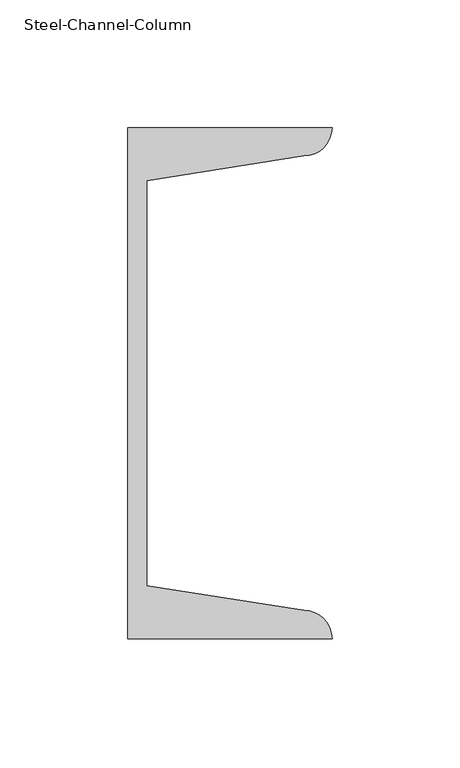
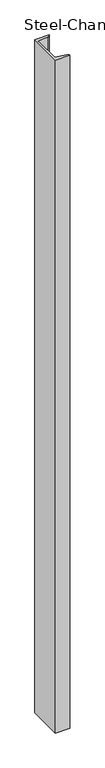
# IFC4 building model written with IfcOpenShell, lengths in millimetres: column geometry, Steel-Channel-Column : CL126_C-200×80x7.5x11.
# Revit data of these elements (continued)
# Project information (continued)
#     -cfd758078946\" /><element revit_id=\"af7cfdda-f71a-4a09-bb03-63e0c16d5d93-001530cf\" ism_id=\"46a5ded9-4fed-43a0-a06e-bb0fce603002\" /><element revit_id=\"af7cfdda-f71a-4a09-bb03-63e0c16d5d93-001530d1\" ism_id=\"62d05a0c-55f2-4c29-a355-b77f91c84c50\" /><element revit_id=\"af7cfdda-f71a-4a09-bb03-63e0c16d5d93-001530d3\" ism_id=\"eac0c420-7041-45a3-ad98-0cab4f5d8155\" /><element revit_id=\"af7cfdda-f71a-4a09-bb03-63e0c16d5d93-001530d5\" ism_id=\"9f5beb51-429a-4c7b-aa2e-ad2efe601ed6\" /><element revit_id=\"af7cfdda-f71a-4a09-bb03-63e0c16d5d93-001530d7\" ism_id=\"4613af3e-a189-4781-a937-106d789655c9\" /><element revit_id=\"af7cfdda-f71a-4a09-bb03-63e0c16d5d93-001530d9\" ism_id=\"71402e21-51c1-43b7-b8cc-75d2aba247eb\" /><element revit_id=\"af7cfdda-f71a-4a09-bb03-63e0c16d5d93-001530db\" ism_id=\"89101b83-9b84-4f11-b026-90cd564a3900\" /><element revit_id=\"af7cfdda-f71a-4a09-bb03-63e0c16d5d93-001530dd\" ism_id=\"37670781-ce23-4ce1-992b-7a400613c37b\" /><element revit_id=\"af7cfdda-f71a-4a09-bb03-63e0c16d5d93-001530df\" ism_id=\"2316856d-18eb-466b-8ab8-114816378db0\" /><element revit_id=\"af7cfdda-f71a-4a09-bb03-63e0c16d5d93-001530e2\" ism_id=\"da4f1597-5b5a-43a6-aa94-e478ffd6cfc7\" /><element revit_id=\"af7cfdda-f71a-4a09-bb03-63e0c16d5d93-001530e5\" ism_id=\"60805764-efb2-4434-8d81-aed3c3ed3c1b\" /><element revit_id=\"af7cfdda-f71a-4a09-bb03-63e0c16d5d93-001530e8\" ism_id=\"34e34ebb-6481-4bfb-b3d0-cb52295ff652\" /><element revit_id=\"af7cfdda-f71a-4a09-bb03-63e0c16d5d93-001530eb\" ism_id=\"dd5c4d73-1406-4c40-a955-5f9c52d01161\" /><element revit_id=\"af7cfdda-f71a-4a09-bb03-63e0c16d5d93-001530ed\" ism_id=\"cf8abc6b-638f-4bd5-8b66-615be032e220\" /><element revit_id=\"af7cfdda-f71a-4a09-bb03-63e0c16d5d93-001530f0\" ism_id=\"56ce8857-0c24-48d5-82f2-459e263998e2\" /><element revit_id=\"af7cfdda-f71a-4a09-bb03-63e0c16d5d93-001530f2\" ism_id=\"a1f000e8-ea08-442b-8a96-da7657653fd5\" /><element revit_id=\"af7cfdda-f71a-4a09-bb03-63e0c16d5d93-001530f4\" ism_id=\"2625e954-f7fb-41eb-b9bd-1b615ef945fc\" /><element revit_id=\"af7cfdda-f71a-4a09-bb03-63e0c16d5d93-001530f6\" ism_id=\"48469362-393c-4deb-bbb2-ad00180a23fb\" /><element revit_id=\"af7cfdda-f71a-4a09-bb03-63e0c16d5d93-001530f8\" ism_id=\"8e650f6f-0906-45a9-8fb8-35680155d6db\" /><element revit_id=\"af7cfdda-f71a-4a09-bb03-63e0c16d5d93-001530fb\" ism_id=\"f84acaf6-20a1-4df6-afed-1dc07fd0b2e9\" /><element revit_id=\"af7cfdda-f71a-4a09-bb03-63e0c16d5d93-001530fe\" ism_id=\"72816c7e-9128-47f4-b46a-ee567a2a03d6\" /><element revit_id=\"af7cfdda-f71a-4a09-bb03-63e0c16d5d93-00153100\" ism_id=\"c95ab0f8-b4bf-4b7c-bd1d-0423c8ac725a\" /><element revit_id=\"af7cfdda-f71a-4a09-bb03-63e0c16d5d93-00153102\" ism_id=\"32fd4119-6673-4973-aef2-b39ef90310e5\" /><element revit_id=\"af7cfdda-f71a-4a09-bb03-63e0c16d5d93-00153104\" ism_id=\"fd2aa4a6-d123-4100-85b9-db27c20cf6bc\" /><element revit_id=\"af7cfdda-f71a-4a09-bb03-63e0c16d5d93-00153106\" ism_id=\"e00fdefa-e77c-4406-9dbe-3c9122259821\" /><element revit_id=\"af7cfdda-f71a-4a09-bb03-63e0c16d5d93-00153108\" ism_id=\"25e5b79e-07c2-4ffa-a7a9-bf039dd2ad78\" /><element revit_id=\"af7cfdda-f71a-4a09-bb03-63e0c16d5d93-0015310b\" ism_id=\"720021d4-ca74-47c0-9c64-7d0854fa39f5\" /><element revit_id=\"af7cfdda-f71a-4a09-bb03-63e0c16d5d93-0015310d\" ism_id=\"ea922120-0cff-4f8d-a5c2-2841c031873e\" /><element revit_id=\"af7cfdda-f71a-4a09-bb03-63e0c16d5d93-0015310f\" ism_id=\"9d07ca73-3a65-44fe-ab61-476d8d1352d1\" /><element revit_id=\"af7cfdda-f71a-4a09-bb03-63e0c16d5d93-00153111\" ism_id=\"68a2fb30-d213-40c7-a166-dad5a20bd269\" /><element revit_id=\"af7cfdda-f71a-4a09-bb03-63e0c16d5d93-00153113\" ism_id=\"06119775-28f9-44f0-a265-5c57029016d1\" /><element revit_id=\"af7cfdda-f71a-4a09-bb03-63e0c16d5d93-00153115\" ism_id=\"ca133383-8253-4d07-aa92-f507fbb2ee47\" /><element revit_id=\"af7cfdda-f71a-4a09-bb03-63e0c16d5d93-00153117\" ism_id=\"6f4a7c07-4bd3-4c99-b1e4-110c964ccc07\" /><element revit_id=\"af7cfdda-f71a-4a09-bb03-63e0c16d5d93-00153119\" ism_id=\"ee1f865b-98a9-4ff1-a84c-52926e8f3566\" /><element revit_id=\"af7cfdda-f71a-4a09-bb03-63e0c16d5d93-0015311b\" ism_id=\"4fd7bd5c-7c46-4e79-a72b-dab4a1d98f33\" /><element revit_id=\"af7cfdda-f71a-4a09-bb03-63e0c16d5d93-0015311e\" ism_id=\"9ca0cac6-aaff-412a-b9c1-a8be985bc44a\" /><element revit_id=\"af7cfdda-f71a-4a09-bb03-63e0c16d5d93-00153121\" ism_id=\"73123639-76b5-46f0-a49e-b26af36d93b1\" /><element revit_id=\"af7cfdda-f71a-4a09-bb03-63e0c16d5d93-00153123\" ism_id=\"f74e8cb9-a93d-4aaa-985b-c0ed9befad19\" /><element revit_id=\"af7cfdda-f71a-4a09-bb03-63e0c16d5d93-00153126\" ism_id=\"5778daa1-b4cb-4cc3-9b7d-323562a47fba\" /><element revit_id=\"af7cfdda-f71a-4a09-bb03-63e0c16d5d93-00153129\" ism_id=\"2d7457d2-8978-4c95-9056-ebbaed3263eb\" /><element revit_id=\"af7cfdda-f71a-4a09-bb03-63e0c16d5d93-0015312c\" ism_id=\"48b420ce-6767-430a-aadc-695c25361a2d\" /><element revit_id=\"af7cfdda-f71a-4a09-bb03-63e0c16d5d93-0015312e\" ism_id=\"fc34038c-136d-4d55-b951-9cc35899fd33\" /><element revit_id=\"af7cfdda-f71a-4a09-bb03-63e0c16d5d93-00153130\" ism_id=\"e7a25938-3b91-4519-a48d-86fdd79489d5\" /><element revit_id=\"af7cfdda-f71a-4a09-bb03-63e0c16d5d93-00153133\" ism_id=\"c81dfd8c-579c-4d77-ab89-bf1f415d9cc6\" /><element revit_id=\"af7cfdda-f71a-4a09-bb03-63e0c16d5d93-00153136\" ism_id=\"5756a4b4-84ca-418c-b9f6-2d2370afca2f\" /><element revit_id=\"af7cfdda-f71a-4a09-bb03-63e0c16d5d93-0015313a\" ism_id=\"09a9cede-a757-4d8e-a722-6140af98bc61\" /><element revit_id=\"af7cfdda-f71a-4a09-bb03-63e0c16d5d93-0015313d\" ism_id=\"ac9b583c-7f63-4351-8b69-3967279b234c\" /><element revit_id=\"af7cfdda-f71a-4a09-bb03-63e0c16d5d93-00153140\" ism_id=\"1a52584d-6b21-4de6-bb42-5b9bdd6f24e9\" /><element revit_id=\"af7cfdda-f71a-4a09-bb03-63e0c16d5d93-00153143\" ism_id=\"6c2e2bc0-8432-4c98-9292-cbb2182bd4b0\" /><element revit_id=\"af7cfdda-f71a-4a09-bb03-63e0c16d5d93-00153145\" ism_id=\"644bb900-7654-42c5-a9b7-996a2197f6d0\" /><element revit_id=\"af7cfdda-f71a-4a09-bb03-63e0c16d5d93-00153148\" ism_id=\"a1bca0bd-75db-464c-b27a-2a69d9b4ad3d\" /><element revit_id=\"af7cfdda-f71a-4a09-bb03-63e0c16d5d93-0015314a\" ism_id=\"ea29955b-34f2-409a-aefa-e6adfe75349e\" /><element revit_id=\"af7cfdda-f71a-4a09-bb03-63e0c16d5d93-0015314d\" ism_id=\"800fef33-e5e1-422c-b708-e9394bbeefcc\" /><element revit_id=\"af7cfdda-f71a-4a09-bb03-63e0c16d5d93-0015314f\" ism_id=\"86259dca-8773-4253-ac56-e71252267c8a\" /><element revit_id=\"af7cfdda-f71a-4a09-bb03-63e0c16d5d93-00153152\" ism_id=\"d15a0ad2-db9f-420d-bea3-41a78a0eb330\" /><element revit_id=\"af7cfdda-f71a-4a09-bb03-63e0c16d5d93-00153155\" ism_id=\"bd27f420-df49-4abe-bd96-8e48e7f4efcb\" /><element revit_id=\"af7cfdda-f71a-4a09-bb03-63e0c16d5d93-00153157\" ism_id=\"5d451f94-860d-4cc3-a4fa-51a9f3126e33\" /><element revit_id=\"af7cfdda-f71a-4a09-bb03-63e0c16d5d93-0015315a\" ism_id=\"4234158a-994a-492b-85da-6108709b7232\" /><element revit_id=\"af7cfdda-f71a-4a09-bb03-63e0c16d5d93-0015315c\" ism_id=\"ca24c92d-986b-417f-812f-024ab15e24c8\" /><element revit_id=\"af7cfdda-f71a-4a09-bb03-63e0c16d5d93-0015315f\" ism_id=\"699ec3b0-0151-4110-b054-14418651f324\" /><element revit_id=\"af7cfdda-f71a-4a09-bb03-63e0c16d5d93-00153161\" ism_id=\"38ecdeac-3d85-48dd-82c1-53fe93f49beb\" /><element revit_id=\"af7cfdda-f71a-4a09-bb03-63e0c16d5d93-00153163\" ism_id=\"1340aefd-b79c-4264-8a49-d0a0504eff8c\" /><element revit_id=\"af7cfdda-f71a-4a09-bb03-63e0c16d5d93-00153165\" ism_id=\"1b6167c2-fb26-4b8d-916b-d835d89896e7\" /><element revit_id=\"af7cfdda-f71a-4a09-bb03-63e0c16d5d93-00153167\" ism_id=\"290d3d83-57eb-4125-aecb-a977a5fcf5ca\" /><element revit_id=\"af7cfdda-f71a-4a09-bb03-63e0c16d5d93-00153169\" ism_id=\"105c9b97-1c70-4237-82ac-8404a3e8e6a6\" /><element revit_id=\"af7cfdda-f71a-4a09-bb03-63e0c16d5d93-0015316c\" ism_id=\"1726c5bb-05e2-4959-9da2-4227f0219f00\" /><element revit_id=\"af7cfdda-f71a-4a09-bb03-63e0c16d5d93-0015316e\" ism_id=\"d919ee9c-caed-4119-b451-e3644db952c8\" /><element revit_id=\"af7cfdda-f71a-4a09-bb03-63e0c16d5d93-00153170\" ism_id=\"1b1fab26-60c4-40ed-b31b-b177eda246ce\" /><element revit_id=\"af7cfdda-f71a-4a09-bb03-63e0c16d5d93-00153172\" ism_id=\"ea9b5221-a1f2-4796-8cca-f7872ab69cbd\" /><element revit_id=\"af7cfdda-f71a-4a09-bb03-63e0c16d5d93-00153174\" ism_id=\"660b40b2-06fb-4b62-b987-28a171e473fe\" /><element revit_id=\"af7cfdda-f71a-4a09-bb03-63e0c16d5d93-00153176\" ism_id=\"767be0d9-c5ba-4ad3-a52d-efd60031fc9a\" /><element revit_id=\"af7cfdda-f71a-4a09-bb03-63e0c16d5d93-00153178\" ism_id=\"6fbe93ce-4ed7-4596-88fc-71dafe48803e\" /><element revit_id=\"af7cfdda-f71a-4a09-bb03-63e0c16d5d93-0015317a\" ism_id=\"27d7b093-4eb7-47aa-b123-5388a6327d7f\" /><element revit_id=\"af7cfdda-f71a-4a09-bb03-63e0c16d5d93-0015317c\" ism_id=\"9073a947-5952-42fe-b37a-cdfed3ca30c7\" /><element revit_id=\"af7cfdda-f71a-4a09-bb03-63e0c16d5d93-0015317e\" ism_id=\"1888f060-aa3c-4494-8f30-a80ca2311216\" /><element revit_id=\"af7cfdda-f71a-4a09-bb03-63e0c16d5d93-00153181\" ism_id=\"c0491dc2-5df2-4c14-b988-e117f6f511a2\" /><element revit_id=\"af7cfdda-f71a-4a09-bb03-63e0c16d5d93-00153184\" ism_id=\"4f44b9aa-c092-46fe-bf9b-2d1be872d419\" /><element revit_id=\"af7cfdda-f71a-4a09-bb03-63e0c16d5d93-00153186\" ism_id=\"eb560801-76cf-40a8-a181-31cd32aca14f\" /><element revit_id=\"af7cfdda-f71a-4a09-bb03-63e0c16d5d93-00153189\" ism_id=\"8d1e5f00-41d5-42c1-9b4f-a8c2eb689a72\" /><element revit_id=\"af7cfdda-f71a-4a09-bb03-63e0c16d5d93-0015318b\" ism_id=\"caf6c2dc-0e9e-46a9-a3e1-71316081ff61\" /><element revit_id=\"af7cfdda-f71a-4a09-bb03-63e0c16d5d93-0015318d\" ism_id=\"4d149f88-f5b9-4943-8765-090324e0a65d\" /><element revit_id=\"af7cfdda-f71a-4a09-bb03-63e0c16d5d93-0015318f\" ism_id=\"75865cf2-3adc-4a52-a778-fc6fb65fcdcb\" /><element revit_id=\"af7cfdda-f71a-4a09-bb03-63e0c16d5d93-00153191\" ism_id=\"f9320017-2083-48f1-8aff-e6ba958fb1c5\" /><element revit_id=\"af7cfdda-f71a-4a09-bb03-63e0c16d5d93-00153193\" ism_id=\"38a61c12-98f2-47b1-843d-8351040e24d2\" /><element revit_id=\"af7cfdda-f71a-4a09-bb03-63e0c16d5d93-00153196\" ism_id=\"af709a9c-b664-480b-be0d-fb01aac630f2\" /><element revit_id=\"af7cfdda-f71a-4a09-bb03-63e0c16d5d93-00153199\" ism_id=\"a4c2867c-ca2a-4112-b86c-4e6563e3dc63\" /><element revit_id=\"14a48413-84c4-4e00-9e64-4f618415469a-0013ce74\" ism_id=\"F2ADF140-E21A-4820-8170-6F63D956DCAD\" /><element revit_id=\"14a48413-84c4-4e00-9e64-4f618415469a-0013ce74\" ism_id=\"B35A310E-4F33-462b-819C-3ADD300C0CEB\" /><element revit_id=\"14a48413-84c4-4e00-9e64-4f618415469a-0013ce74\" ism_id=\"711054EC-0DB2-46e3-AD20-004560300C00\" /><element revit_id=\"14a48413-84c4-4e00-9e64-4f618415469a-0013ce6e\" ism_id=\"B5C54EC9-8EBD-4860-AB72-EF5791AED394\" /><element revit_id=\"14a48413-84c4-4e00-9e64-4f618415469a-0013e793\" ism_id=\"0A7B8D02-9EA4-4aa9-A41A-E30BB5B6B6C5\" /><element revit_id=\"14a48413-84c4-4e00-9e64-4f618415469a-0013e793\" ism_id=\"714BBD27-DB58-47da-B54C-5806291C2D3C\" /><element revit_id=\"14a48413-84c4-4e00-9e64-4f618415469a-0013e793\" ism_id=\"F36E62C1-13EE-4807-A3C1-899E23E0BEDE\" /><element revit_id=\"14a48413-84c4-4e00-9e64-4f618415469a-0013e793\" ism_id=\"F5448801-679E-44d6-8F46-E676344F8165\" /><element revit_id=\"14a48413-84c4-4e00-9e64-4f618415469a-0013e793\" ism_id=\"846DCB0C-E06B-4978-9D43-E1CC0FDE7595\" /><element revit_id=\"14a48413-84c4-4e00-9e64-4f618415469a-0013e793\" ism_id=\"2ADF82B8-986D-4f44-85DE-89D921292160\" /><element revit_id=\"14a48413-84c4-4e00-9e64-4f618415469a-0013e793\" ism_id=\"7AF371ED-051B-4a30-8826-11F11C212B73\" /><element revit_id=\"14a48413-84c4-4e00-9e64-4f618415469a-0013e793\" ism_id=\"2FE74006-ADDA-412f-A522-853919E62B4D\" /><element revit_id=\"14a48413-84c4-4e00-9e64-4f618415469a-0013e793\" ism_id=\"09B63641-D581-4a6c-A18E-54C17EC989A4\" /><element revit_id=\"14a48413-84c4-4e00-9e64-4f618415469a-0013e793\" ism_id=\"0DD6B52A-77D0-45a1-82B1-8236ED57078C\" /><element revit_id=\"14a48413-84c4-4e00-9e64-4f618415469a-0013e793\" ism_id=\"35D311D2-DEB8-4469-97DE-110B6DF5B84D\" /><element revit_id=\"14a48413-84c4-4e00-9e64-4f618415469a-0013e79
#     3\" ism_id=\"0D3CCDE5-CFF9-431b-A4BD-01BF6636D6BD\" /><element revit_id=\"14a48413-84c4-4e00-9e64-4f618415469a-0013e793\" ism_id=\"C62B2A5B-024A-47ac-B030-C17A67E64A7B\" /><element revit_id=\"14a48413-84c4-4e00-9e64-4f618415469a-0013e793\" ism_id=\"944C6E43-E607-48c3-8358-9E6CB88346E7\" /><element revit_id=\"14a48413-84c4-4e00-9e64-4f618415469a-0013e793\" ism_id=\"A4B1F42D-B1C2-4ad2-8AD6-DB0D5E05998D\" /><element revit_id=\"14a48413-84c4-4e00-9e64-4f618415469a-0013e793\" ism_id=\"007E6C70-1139-4b48-B003-C76FAD4C249A\" /><element revit_id=\"14a48413-84c4-4e00-9e64-4f618415469a-0013e793\" ism_id=\"9941AC94-F03A-464c-9912-04590E0C31E0\" /><element revit_id=\"14a48413-84c4-4e00-9e64-4f618415469a-0013e793\" ism_id=\"CFD98B8D-8FF4-4e71-A909-0FE7DBCE924E\" /><element revit_id=\"14a48413-84c4-4e00-9e64-4f618415469a-0013e793\" ism_id=\"58262161-98E6-45c8-B2BD-4508105FF662\" /><element revit_id=\"14a48413-84c4-4e00-9e64-4f618415469a-0013e793\" ism_id=\"66AB4841-610A-4883-97F7-1282A56484E1\" /><element revit_id=\"14a48413-84c4-4e00-9e64-4f618415469a-0013e793\" ism_id=\"D2B324BE-BBD6-49da-9730-60EA7AD4D3A0\" /><element revit_id=\"14a48413-84c4-4e00-9e64-4f618415469a-0013e793\" ism_id=\"92A8ECE7-C053-46b1-92ED-F2C041617E7B\" /><element revit_id=\"14a48413-84c4-4e00-9e64-4f618415469a-0013e793\" ism_id=\"B4C4BDB0-65C4-4016-9C78-DBD77E229523\" /><element revit_id=\"14a48413-84c4-4e00-9e64-4f618415469a-0013e793\" ism_id=\"57270646-162F-4c83-BDB7-A5FBEA9120BD\" /><element revit_id=\"14a48413-84c4-4e00-9e64-4f618415469a-0013e793\" ism_id=\"BDEF733F-00AA-4eee-B6C6-50229FC1D236\" /><element revit_id=\"14a48413-84c4-4e00-9e64-4f618415469a-0013e793\" ism_id=\"84A94E1E-3074-40f4-9690-97191755F019\" /><element revit_id=\"14a48413-84c4-4e00-9e64-4f618415469a-0013e793\" ism_id=\"8A7D913D-7967-4718-912D-B83DF0AD2EDD\" /><element revit_id=\"14a48413-84c4-4e00-9e64-4f618415469a-0013e793\" ism_id=\"83553D70-90FA-469c-B5C3-EF03F3FC6475\" /><element revit_id=\"14a48413-84c4-4e00-9e64-4f618415469a-0013e793\" ism_id=\"6880C1E4-C50B-4c1b-B61C-23F2D8C46873\" /><element revit_id=\"14a48413-84c4-4e00-9e64-4f618415469a-0013e793\" ism_id=\"08594C43-CD40-47de-A3BA-8BFB47F64994\" /><element revit_id=\"14a48413-84c4-4e00-9e64-4f618415469a-0013e793\" ism_id=\"7D2E11FA-A5E1-4434-B9BE-AABA1A16CA03\" /><element revit_id=\"14a48413-84c4-4e00-9e64-4f618415469a-0013e793\" ism_id=\"D892DFA4-5441-4ad2-A390-253492293B1B\" /><element revit_id=\"14a48413-84c4-4e00-9e64-4f618415469a-0013e793\" ism_id=\"E5A32FE6-89C4-49f1-B3B9-1CABE7C48A4D\" /><element revit_id=\"14a48413-84c4-4e00-9e64-4f618415469a-0013e793\" ism_id=\"8AE872C2-5DBE-47c5-934B-7E964A84B589\" /><element revit_id=\"14a48413-84c4-4e00-9e64-4f618415469a-0013e793\" ism_id=\"3C847B60-488A-4604-A400-16A3A65E919B\" /><element revit_id=\"14a48413-84c4-4e00-9e64-4f618415469a-0013e793\" ism_id=\"DBEC432A-3F7B-4266-AD99-2A937DC70BCF\" /><element revit_id=\"14a48413-84c4-4e00-9e64-4f618415469a-0013e793\" ism_id=\"59403DD6-7A51-48aa-A3BE-962457E6F10E\" /><element revit_id=\"14a48413-84c4-4e00-9e64-4f618415469a-0013e793\" ism_id=\"11CDDF5D-38B6-43b2-A291-FC188BE232BC\" /><element revit_id=\"14a48413-84c4-4e00-9e64-4f618415469a-0013e793\" ism_id=\"10BF2843-EFC9-4136-933C-5B270D970277\" /><element revit_id=\"14a48413-84c4-4e00-9e64-4f618415469a-0013e793\" ism_id=\"E1B09A9C-F6C6-47d9-976B-E313C0E3F52B\" /><element revit_id=\"14a48413-84c4-4e00-9e64-4f618415469a-0013e793\" ism_id=\"A3A22EC3-26C8-4588-A0AB-AFAE02DF267E\" /><element revit_id=\"14a48413-84c4-4e00-9e64-4f618415469a-0013e793\" ism_id=\"114828FC-BDC1-4343-9119-BCB5395DAA64\" /><element revit_id=\"14a48413-84c4-4e00-9e64-4f618415469a-0013e793\" ism_id=\"797626F9-3558-4623-826F-15FB93088CB3\" /><element revit_id=\"14a48413-84c4-4e00-9e64-4f618415469a-0013e793\" ism_id=\"4BF369CD-DF09-4346-96CB-C6C6380A2599\" /><element revit_id=\"14a48413-84c4-4e00-9e64-4f618415469a-0013e793\" ism_id=\"722B46BA-61C4-44a1-9ECF-325B60B6688D\" /><element revit_id=\"14a48413-84c4-4e00-9e64-4f618415469a-0013e793\" ism_id=\"C33DBE84-19C1-4379-AB6E-A41F7420F18C\" /><element revit_id=\"14a48413-84c4-4e00-9e64-4f618415469a-0013e793\" ism_id=\"1F2D3B75-66F2-4d88-A1DD-647969477B86\" /><element revit_id=\"14a48413-84c4-4e00-9e64-4f618415469a-0013e793\" ism_id=\"DFBF96B2-410A-4f39-80C4-D8CF78561C93\" /><element revit_id=\"14a48413-84c4-4e00-9e64-4f618415469a-0013e793\" ism_id=\"D6793CD3-AB64-417c-9C28-8B18A0A2D336\" /><element revit_id=\"14a48413-84c4-4e00-9e64-4f618415469a-0013e793\" ism_id=\"90884AC0-EA00-4caa-86E1-E6B886FD90ED\" /><element revit_id=\"14a48413-84c4-4e00-9e64-4f618415469a-0013e793\" ism_id=\"64BC7B89-F7C8-4dae-A5C8-F10DF9E5F6BA\" /><element revit_id=\"14a48413-84c4-4e00-9e64-4f618415469a-0013e793\" ism_id=\"D82E4D85-2728-40e5-9F60-1C7FB2990D78\" /><element revit_id=\"14a48413-84c4-4e00-9e64-4f618415469a-0013e793\" ism_id=\"1E6D05B9-BF84-4669-AA27-948ADA1D511E\" /><element revit_id=\"14a48413-84c4-4e00-9e64-4f618415469a-0013e793\" ism_id=\"73608CB2-EB94-466e-883D-814030EF49D6\" /><element revit_id=\"14a48413-84c4-4e00-9e64-4f618415469a-0013e793\" ism_id=\"4EAF07EF-4E08-4065-9F08-BF69D4413867\" /><element revit_id=\"14a48413-84c4-4e00-9e64-4f618415469a-0013e0e9\" ism_id=\"05D74241-6318-4cac-95F5-7B878260D5B5\" /></element_binding><reinforcement_properties /><operation_settings><coordinate_mapping x=\"0\" y=\"0\" z=\"0\" /></operation_settings></ism>"
#   Building Name = "FIRE WATER PUMP BUILDING"
#   Project Status = "Project Status"
#   Client Name = "현대엔지니어링"
#   Project Address = "서울시 종로구 율곡로 75(계동)"
#   Project Name = "TAKHIATASH POWER PLANT EFFICIENCY IMPROVEMENT PROJECT / 우즈베키스탄"
#   Project Number = "BEUZ1602"
#   F01) Building Name = "FIRE WATER PUMP BUILDING"
#   F11) Project Building Tag_Type-1 = "BI aWBS"
#   F12) Project Building Tag_Type-2 = "BI aWBS"
#   F13) Project Facility Code = "621"
#   F21) Structural Type = "STEEL"
#   F31) Standard Building Code = "E204"
#   F41) Discipline = "Architecture"
#   F51) Plan Start Date-Engineering = "2018-01-01"
#   F52) Plan Finish Date-Engineering = "2018-09-13"
#   F53) Duration = "255"
#   F61) Plan Start Date-Construction = "2018-09-14"
#   F62) Plan Finish Date-Construction = "2019-12-02"
#   F63) Duration = "444"
#   F91) Plant Type = "2GTG+2STG+1HRSG"
#   F92) KKS Structures, Building = "UAB"
#   P01) Project Name = "TAKHIATASH POWER PLANT EFFICIENCY IMPROVEMENT PROJECT / 우즈베키스탄"
#   P02) Project Configuration = "2 GTG + 2 HRSG + 2STG, 2 x 250MW"
#   P03) Project Abbreviation = "UTCC"
#   P04) Project Code = "BEUZ1602"
#   P05) Project Stage = "실행"
#   P06) Project Location = "Takhiatash / Uzbekistan"
#   P07) Project Owner = "우즈베키스탄 전력청"
#   P08) Project O.E = "GAS Natural Fenosa"
#   P09) Project Schedule = "2017.10.01 ~ 2020.08.08"
#   P10) Basic Wind Speed = "48m/sec_ASCE7-05"
#   P11) Seismic = "SDS_0.15_ASCE7-05"
#   P12) Soil = "SD_ASCE7-05"
#   P13) Soil Capacity = "400 kN/m2_Soil Replacement"
#   P14) Pile Capacity = "1000 kN_D600 Board Pile"
# Type "Steel-Channel-Column : CL126_C-200×80x7.5x11"
#   Assembly Code = "B10"
#   x = 22.1 mm
#   Section Area = 31.33 cm²
#   Mass per Unit Length = 24.60 kg/m
#   bf = 80 mm
#   d = 200 mm
#   tf = 11 mm
#   tw = 7.5 mm
#   hec_material4 [instance default] = none
#   hec_material3 [instance default] = none
#   hec_material2 [instance default] = none
#   hec_material1 [instance default] = none
#   Structural Material [instance default] = Steel, 45-345
# Element 1 (IfcColumn, "Steel-Channel-Column : CL126_C-200×80x7.5x11")
#   Materials on its faces: "Steel, 45-345"
# Materials
#   "Steel, 45-345": class "Metal", colour RGB 189 187 185, transparency 0, Description = "Steel 345 MPa", Cost = 0
